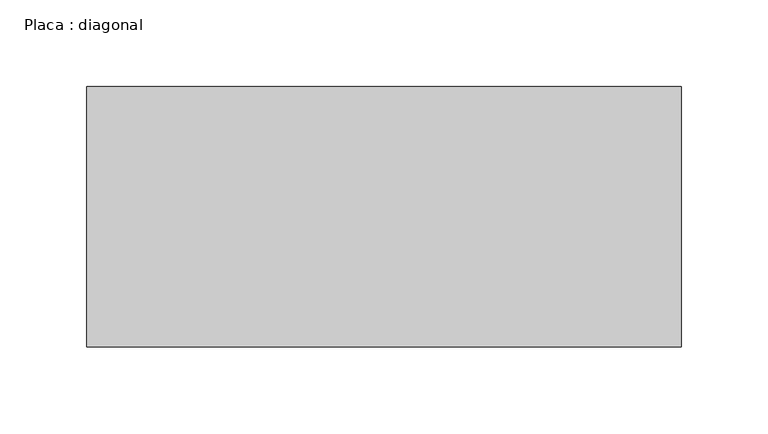
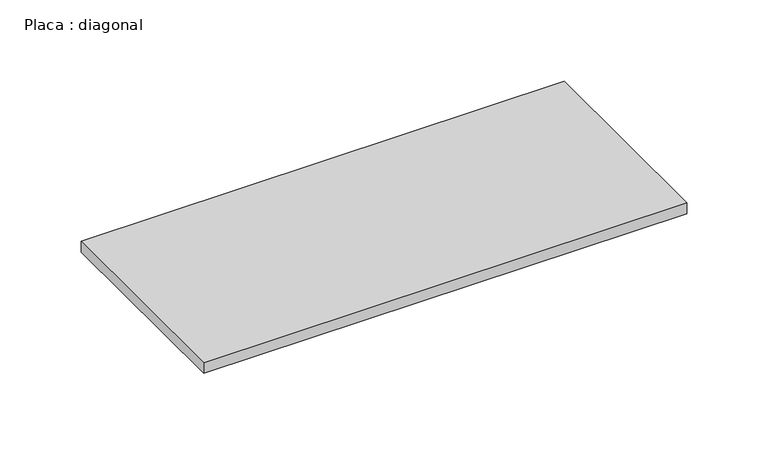
"""IFC4 building model written with IfcOpenShell, lengths in millimetres: beam geometry, Placa : diagonal."""

from ifc_helpers import new_model, si_unit, frame, origin, place, context, project, spatial, polyline, outline, extrude, source, transform, mapped, element, save


def placa_diagonal_c1c8cf8f(model_context):
    return source(origin(), model_context, "Body", "SweptSolid", [
        extrude(outline(polyline([(171.6122393, 75.0), (171.6122393, -75.0), (-170.6977761, -75.0), (-170.6977761, 75.0), (171.6122393, 75.0)])), frame((0.0, 0.0, -4.0), z_axis=(0.0, 0.0, 1.0), x_axis=(1.0, 0.0, 0.0)), (0.0, 0.0, 1.0), 8.0),
    ])


if __name__ == "__main__":
    model = new_model("IFC4")
    model_context = context("Model", 3, world=origin())
    ifc_project = project(units=[si_unit("LENGTHUNIT", "METRE", prefix="MILLI")], contexts=[model_context])
    site = spatial("IfcSite", under=ifc_project)
    building = spatial("IfcBuilding", under=site)
    placement = place(None, origin())
    placa_diagonal_shape = placa_diagonal_c1c8cf8f(model_context)
    element("IfcBeam", 1, ObjectType="Placa : diagonal", at=placement, inside=building, context=model_context, shape_type="MappedRepresentation", body=[
        mapped(placa_diagonal_shape, transform((0.0, 0.0, 0.0), x_axis=(1.0, 0.0, 0.0), y_axis=(0.0, 1.0, 0.0), z_axis=(0.0, 0.0, 1.0))),
    ])
    save(model, "model.ifc")

# Revit data of these elements
# Type "Placa : diagonal"
#   W = 0
#   Length [instance default] = 1.50 m
#   b = 0.15 m
#   d = 0.008 m
#   A = 0 m²
#   Structural Material [instance default] = Aço, 45-345
# Element 1 (IfcBeam, "Placa : diagonal")
#   Materials on its faces: "Aço, 45-345"
# Materials
#   "Aço, 45-345": class "Metal", colour RGB 247 247 247, transparency 0, Description = "Aço 345 MPa", Cost = 0
